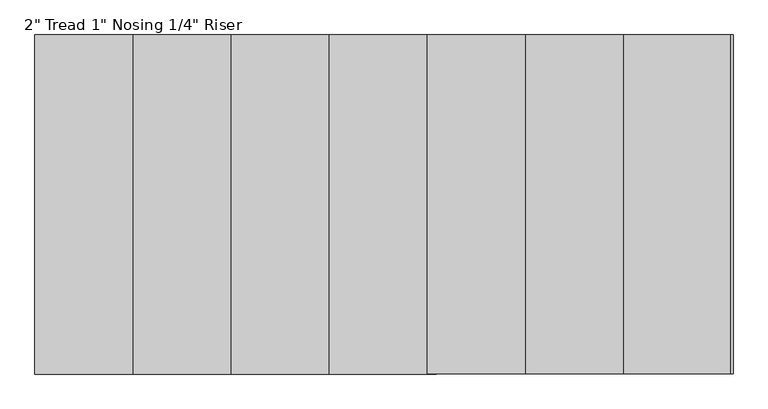
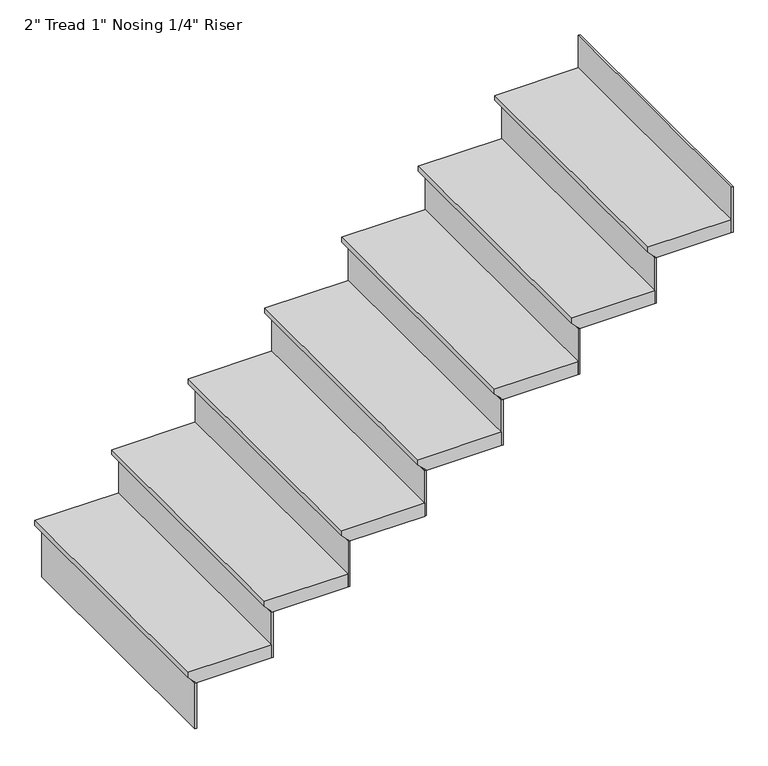
"""IFC4 building model written with IfcOpenShell, lengths in millimetres: stair flight geometry."""

from ifc_helpers import new_model, si_unit, frame, origin, place, context, project, spatial, polyline, outline, extrude, source, transform, mapped, element, save


def stair_flight_08fced55(model_context):
    return source(origin(), model_context, "Body", "SweptSolid", [
        extrude(outline(polyline([(267973.96875, 25112.6590778), (267973.96875, 24807.8590778), (267954.91875, 24807.8590778), (267929.51875, 24833.2590778), (267923.16875, 24833.2590778), (267923.16875, 25112.6590778), (267973.96875, 25112.6590778)])), frame((0.0, 25735.6156612, 0.0), z_axis=(0.0, 1.0, 0.0), x_axis=(0.0, 0.0, 1.0)), (0.0, 0.0, 1.0), 965.2),
        extrude(outline(polyline([(24839.6090778, 25735.6156612), (24833.2590778, 25735.6156612), (24833.2590778, 26700.8156612), (24839.6090778, 26700.8156612), (24839.6090778, 25735.6156612)])), frame((0.0, 0.0, 267747.75), z_axis=(0.0, 0.0, 1.0), x_axis=(1.0, 0.0, 0.0)), (0.0, 0.0, 1.0), 175.41875),
        extrude(outline(polyline([(25119.0090778, 25735.6156612), (25112.6590778, 25735.6156612), (25112.6590778, 26700.8156612), (25119.0090778, 26700.8156612), (25119.0090778, 25735.6156612)])), frame((0.0, 0.0, 267923.16875), z_axis=(0.0, 0.0, 1.0), x_axis=(1.0, 0.0, 0.0)), (0.0, 0.0, 1.0), 175.41875),
        extrude(outline(polyline([(268149.3875, 25392.0590778), (268149.3875, 25087.2590778), (268130.3375, 25087.2590778), (268104.9375, 25112.6590778), (268098.5875, 25112.6590778), (268098.5875, 25392.0590778), (268149.3875, 25392.0590778)])), frame((0.0, 25735.6156612, 0.0), z_axis=(0.0, 1.0, 0.0), x_axis=(0.0, 0.0, 1.0)), (0.0, 0.0, 1.0), 965.2),
        extrude(outline(polyline([(25398.4090778, 25735.6156612), (25392.0590778, 25735.6156612), (25392.0590778, 26700.8156612), (25398.4090778, 26700.8156612), (25398.4090778, 25735.6156612)])), frame((0.0, 0.0, 268098.5875), z_axis=(0.0, 0.0, 1.0), x_axis=(1.0, 0.0, 0.0)), (0.0, 0.0, 1.0), 175.41875),
        extrude(outline(polyline([(268324.80625, 25671.4590778), (268324.80625, 25366.6590778), (268305.75625, 25366.6590778), (268280.35625, 25392.0590778), (268274.00625, 25392.0590778), (268274.00625, 25671.4590778), (268324.80625, 25671.4590778)])), frame((0.0, 25735.6156612, 0.0), z_axis=(0.0, 1.0, 0.0), x_axis=(0.0, 0.0, 1.0)), (0.0, 0.0, 1.0), 965.2),
        extrude(outline(polyline([(25677.8090778, 25735.6156612), (25671.4590778, 25735.6156612), (25671.4590778, 26700.8156612), (25677.8090778, 26700.8156612), (25677.8090778, 25735.6156612)])), frame((0.0, 0.0, 268274.00625), z_axis=(0.0, 0.0, 1.0), x_axis=(1.0, 0.0, 0.0)), (0.0, 0.0, 1.0), 175.41875),
        extrude(outline(polyline([(268500.225, 25950.8590778), (268500.225, 25646.0590778), (268481.175, 25646.0590778), (268455.775, 25671.4590778), (268449.425, 25671.4590778), (268449.425, 25950.8590778), (268500.225, 25950.8590778)])), frame((0.0, 25735.6156612, 0.0), z_axis=(0.0, 1.0, 0.0), x_axis=(0.0, 0.0, 1.0)), (0.0, 0.0, 1.0), 965.2),
        extrude(outline(polyline([(25957.2090778, 25735.6156612), (25950.8590778, 25735.6156612), (25950.8590778, 26700.8156612), (25957.2090778, 26700.8156612), (25957.2090778, 25735.6156612)])), frame((0.0, 0.0, 268449.425), z_axis=(0.0, 0.0, 1.0), x_axis=(1.0, 0.0, 0.0)), (0.0, 0.0, 1.0), 175.41875),
        extrude(outline(polyline([(268675.64375, 26230.2590778), (268675.64375, 25925.4590778), (268656.59375, 25925.4590778), (268631.19375, 25950.8590778), (268624.84375, 25950.8590778), (268624.84375, 26230.2590778), (268675.64375, 26230.2590778)])), frame((0.0, 25735.6156612, 0.0), z_axis=(0.0, 1.0, 0.0), x_axis=(0.0, 0.0, 1.0)), (0.0, 0.0, 1.0), 965.2),
        extrude(outline(polyline([(26236.6090778, 25735.6156612), (26230.2590778, 25735.6156612), (26230.2590778, 26700.8156612), (26236.6090778, 26700.8156612), (26236.6090778, 25735.6156612)])), frame((0.0, 0.0, 268624.84375), z_axis=(0.0, 0.0, 1.0), x_axis=(1.0, 0.0, 0.0)), (0.0, 0.0, 1.0), 175.41875),
        extrude(outline(polyline([(268851.0625, 26509.6590778), (268851.0625, 26204.8590778), (268832.0125, 26204.8590778), (268806.6125, 26230.2590778), (268800.2625, 26230.2590778), (268800.2625, 26509.6590778), (268851.0625, 26509.6590778)])), frame((0.0, 25735.6156612, 0.0), z_axis=(0.0, 1.0, 0.0), x_axis=(0.0, 0.0, 1.0)), (0.0, 0.0, 1.0), 965.2),
        extrude(outline(polyline([(26516.0090778, 25735.6156612), (26509.6590778, 25735.6156612), (26509.6590778, 26700.8156612), (26516.0090778, 26700.8156612), (26516.0090778, 25735.6156612)])), frame((0.0, 0.0, 268800.2625), z_axis=(0.0, 0.0, 1.0), x_axis=(1.0, 0.0, 0.0)), (0.0, 0.0, 1.0), 175.41875),
        extrude(outline(polyline([(26795.4090778, 25735.6156612), (26789.0590778, 25735.6156612), (26789.0590778, 26700.8156612), (26795.4090778, 26700.8156612), (26795.4090778, 25735.6156612)])), frame((0.0, 0.0, 268975.68125), z_axis=(0.0, 0.0, 1.0), x_axis=(1.0, 0.0, 0.0)), (0.0, 0.0, 1.0), 175.41875),
        extrude(outline(polyline([(269026.48125, 26789.0590778), (269026.48125, 26484.2590778), (269007.43125, 26484.2590778), (268982.03125, 26509.6590778), (268975.68125, 26509.6590778), (268975.68125, 26789.0590778), (269026.48125, 26789.0590778)])), frame((0.0, 25735.6156612, 0.0), z_axis=(0.0, 1.0, 0.0), x_axis=(0.0, 0.0, 1.0)), (0.0, 0.0, 1.0), 965.2),
    ])


if __name__ == "__main__":
    model = new_model("IFC4")
    model_context = context("Model", 3, world=origin())
    ifc_project = project(units=[si_unit("LENGTHUNIT", "METRE", prefix="MILLI")], contexts=[model_context])
    site = spatial("IfcSite", under=ifc_project)
    building = spatial("IfcBuilding", under=site)
    placement = place(None, origin())
    stair_flight_shape = stair_flight_08fced55(model_context)
    element("IfcStairFlight", 1, ObjectType="2\" Tread 1\" Nosing 1/4\" Riser", at=placement, inside=building, context=model_context, shape_type="MappedRepresentation", body=[
        mapped(stair_flight_shape, transform((0.0, 0.0, 0.0), x_axis=(1.0, 0.0, 0.0), y_axis=(0.0, 1.0, 0.0), z_axis=(0.0, 0.0, 1.0))),
    ])
    save(model, "model.ifc")

# Revit data of these elements
# Element 1 (IfcStairFlight, "2\" Tread 1\" Nosing 1/4\" Riser")
#   Materials on its faces: "SLOTTED WOOD FENCE (THERMALLY MODIFIED WOOD: ARBOR WOOD)\n(EXTERIOR STAIN : PENOFIN VERDE EXT. STAIN - COLOR: CEDAR)"
# Materials
#   "SLOTTED WOOD FENCE (THERMALLY MODIFIED WOOD: ARBOR WOOD)\n(EXTERIOR STAIN : PENOFIN VERDE EXT. STAIN - COLOR: CEDAR)": class "Wood", colour RGB 164 134 123, transparency 0, Description = "Pinus Echinata", Cost = 0
